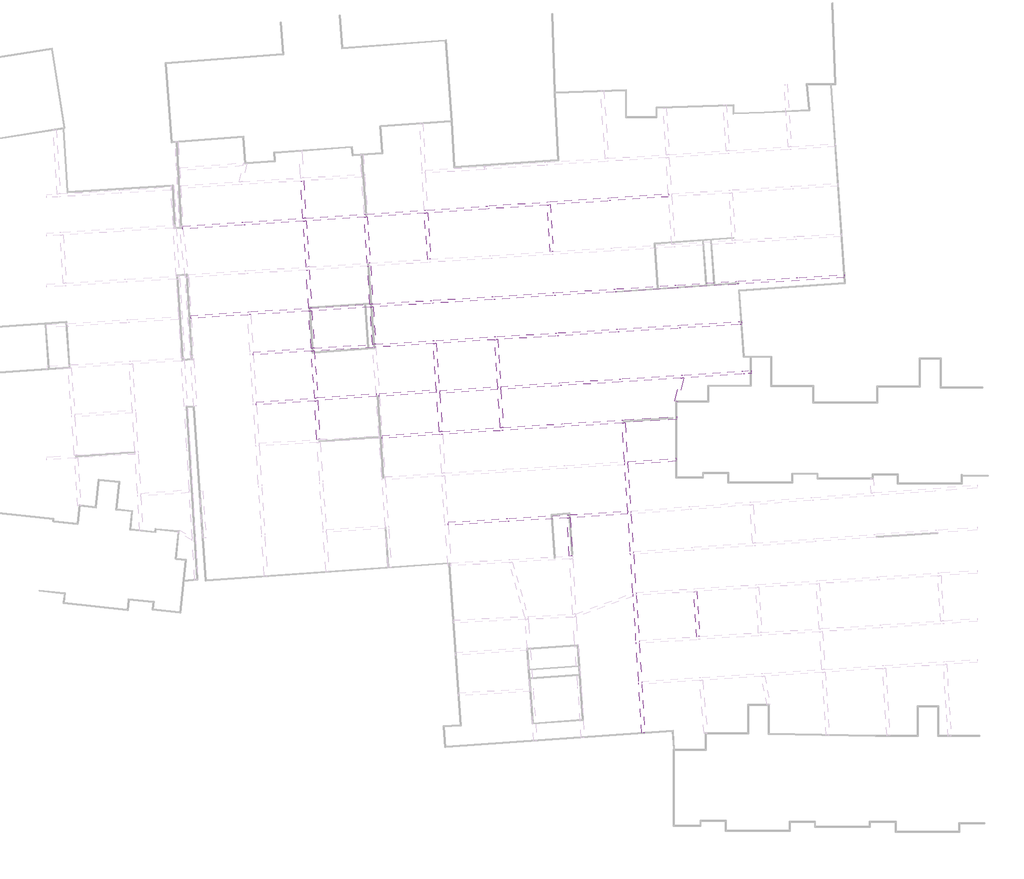
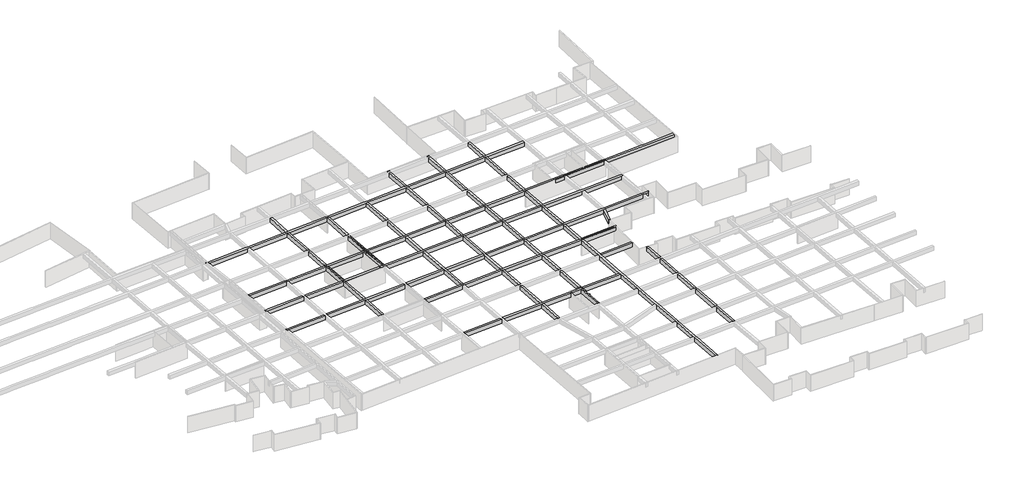
# One storey, part 13 of 14: 27 beams.
"""IFC4 building model written with IfcOpenShell, lengths in millimetres."""

from ifc_helpers import new_model, si_unit, frame, origin, place, context, project, spatial, polyline, outline, extrude, faceted_brep, element, save

model = new_model("IFC4")

# Units and contexts
model_context = context("Model", 3, world=origin())
ifc_project = project(units=[si_unit("LENGTHUNIT", "METRE", prefix="MILLI")], contexts=[model_context])

# Site, building, storey
site = spatial("IfcSite", under=ifc_project)
building = spatial("IfcBuilding", under=site)
storey = spatial("IfcBuildingStorey", under=building, Name="户型图", Elevation=0.0)

# Beams
placement = place(None, origin())
element("IfcBeam", 1, ObjectType="混凝土 - 矩形梁 : KL_beam", at=placement, inside=storey, context=model_context, shape_type="Brep", body=[
    faceted_brep([(-138257.4280169, -132256.5266916, 3300.0), (-138210.5692457, -132654.2910271, 3300.0), (-130469.1405666, -132138.3296148, 3300.0), (-130070.0241354, -132111.7287526, 3300.0), (-122474.0579494, -131605.462325, 3300.0), (-122074.9434283, -131578.8615901, 3300.0), (-114428.1793907, -131069.2095173, 3300.0), (-114029.0614384, -131042.6085537, 3300.0), (-106557.1829705, -130544.6124955, 3300.0), (-106158.0684495, -130518.0117606, 3300.0), (-98469.0899467, -130005.5461199, 3300.0), (-98069.9743702, -129978.9453146, 3300.0), (-90486.7784169, -129473.5300151, 3300.0), (-90087.6628405, -129446.9292099, 3300.0), (-82518.8955366, -128942.4755709, 3300.0), (-82119.7795402, -128915.8747377, 3300.0), (-74549.1899952, -128411.2996475, 3300.0), (-74577.0927331, -128012.2719042, 3300.0), (-82145.2950928, -128516.6878899, 3300.0), (-82544.4110892, -128543.2887232, 3300.0), (-90113.3457028, -129047.7535132, 3300.0), (-90512.4612793, -129074.3543185, 3300.0), (-98095.6572325, -129579.7696179, 3300.0), (-98494.772809, -129606.3704232, 3300.0), (-106181.8169664, -130118.707141, 3300.0), (-106580.971679, -130145.3105546, 3300.0), (-114054.8364044, -130643.4389957, 3300.0), (-114453.9509255, -130670.0397306, 3300.0), (-122098.6919453, -131179.5569705, 3300.0), (-122497.8466579, -131206.1603841, 3300.0), (-130095.3900507, -131712.5319316, 3300.0), (-130494.5064819, -131739.1327938, 3300.0), (-138244.7036771, -132255.6786223, 3300.0), (-138210.5692457, -132654.2910271, 2500.0), (-130469.1405666, -132138.3296148, 2500.0), (-130070.0241354, -132111.7287526, 2500.0), (-122474.0579494, -131605.462325, 2500.0), (-122074.9434283, -131578.8615901, 2500.0), (-114428.1793907, -131069.2095173, 2500.0), (-114029.0614384, -131042.6085537, 2500.0), (-106557.1829705, -130544.6124955, 2500.0), (-106158.0684495, -130518.0117606, 2500.0), (-98469.0899467, -130005.5461199, 2500.0), (-98069.9743702, -129978.9453146, 2500.0), (-90486.7784169, -129473.5300151, 2500.0), (-90087.6628405, -129446.9292099, 2500.0), (-82518.8955366, -128942.4755709, 2500.0), (-82119.7795402, -128915.8747377, 2500.0), (-74549.1899952, -128411.2996475, 2500.0), (-138257.4280169, -132256.5266916, 2500.0), (-138244.7036771, -132255.6786223, 2500.0), (-130494.5064819, -131739.1327938, 2500.0), (-130095.3900507, -131712.5319316, 2500.0), (-122497.8466579, -131206.1603841, 2500.0), (-122098.6919453, -131179.5569705, 2500.0), (-114453.9509255, -130670.0397306, 2500.0), (-114054.8364044, -130643.4389957, 2500.0), (-106580.971679, -130145.3105546, 2500.0), (-106181.8169664, -130118.707141, 2500.0), (-98494.772809, -129606.3704232, 2500.0), (-98095.6572325, -129579.7696179, 2500.0), (-90512.4612793, -129074.3543185, 2500.0), (-90113.3457028, -129047.7535132, 2500.0), (-82544.4110892, -128543.2887232, 2500.0), (-82145.2950928, -128516.6878899, 2500.0), (-74577.0927331, -128012.2719042, 2500.0), (-138657.0563303, -132283.1616705, 2500.0), (-138657.0563303, -132283.1616705, 3300.0), (-138643.8583896, -132282.2820359, 3300.0), (-138643.8583896, -132282.2820359, 2500.0), (-138654.6809564, -132303.3252176, 2500.0), (-138654.6809564, -132303.3252176, 3300.0)], [[[0, 1, 2, 3, 4, 5, 6, 7, 8, 9, 10, 11, 12, 13, 14, 15, 16, 17, 18, 19, 20, 21, 22, 23, 24, 25, 26, 27, 28, 29, 30, 31, 32]], [[1, 33, 34, 35, 36, 37, 38, 39, 40, 41, 42, 43, 44, 45, 46, 47, 48, 16, 15, 14, 13, 12, 11, 10, 9, 8, 7, 6, 5, 4, 3, 2]], [[33, 49, 50, 51, 52, 53, 54, 55, 56, 57, 58, 59, 60, 61, 62, 63, 64, 65, 48, 47, 46, 45, 44, 43, 42, 41, 40, 39, 38, 37, 36, 35, 34]], [[66, 67, 68, 0, 32, 31, 30, 29, 28, 27, 26, 25, 24, 23, 22, 21, 20, 19, 18, 17, 65, 64, 63, 62, 61, 60, 59, 58, 57, 56, 55, 54, 53, 52, 51, 50, 49, 69]], [[67, 66, 70, 71]], [[0, 49, 33, 1]], [[49, 0, 71, 70]], [[67, 71, 0, 68]], [[70, 66, 69, 49]], [[17, 16, 48, 65]]]),
])
element("IfcBeam", 2, ObjectType="混凝土 - 矩形梁 : KL_beam", at=placement, inside=storey, context=model_context, shape_type="Brep", body=[
    faceted_brep([(-51536.7180221, -138597.7306063, 3300.0), (-51511.7724706, -138996.9519979, 3300.0), (-51511.7724706, -138996.9519979, 2500.0), (-51536.7180221, -138597.7306063, 2500.0), (-57425.127004, -138965.6708341, 3300.0), (-57824.3483955, -138990.6163857, 3300.0), (-65411.3764652, -139464.6956904, 3300.0), (-65810.6088137, -139489.6419266, 3300.0), (-73340.6382748, -139960.1596443, 3300.0), (-73739.8706232, -139985.1058805, 3300.0), (-81381.7257688, -140462.611083, 3300.0), (-81780.9475672, -140487.5566599, 3300.0), (-89346.8943039, -140960.3186869, 3300.0), (-89746.1163762, -140985.2642809, 3300.0), (-97331.3357508, -141459.2305685, 3300.0), (-97730.5578232, -141484.1761625, 3300.0), (-105395.2598308, -141963.1089628, 3300.0), (-105794.4846545, -141988.0547288, 3300.0), (-113315.7632998, -142458.0256473, 3300.0), (-113714.9846914, -142482.9711989, 3300.0), (-121338.0144185, -142959.3000855, 3300.0), (-121737.2358101, -142984.245637, 3300.0), (-129348.9364688, -143459.8666211, 3300.0), (-129748.1580815, -143484.8121864, 3300.0), (-137166.9194829, -143948.3772629, 3300.0), (-137141.9739314, -144347.5986544, 3300.0), (-129722.7922736, -143884.007318, 3300.0), (-129323.5706608, -143859.0617527, 3300.0), (-121712.2902585, -143383.4670286, 3300.0), (-121313.068867, -143358.521477, 3300.0), (-113688.5657164, -142882.1005228, 3300.0), (-113289.333368, -142857.1542866, 3300.0), (-105767.8836909, -142387.1726811, 3300.0), (-105368.6588672, -142362.2269151, 3300.0), (-97704.874985, -141883.3514844, 3300.0), (-97305.6529126, -141858.4058903, 3300.0), (-89720.433538, -141384.4396028, 3300.0), (-89321.2114657, -141359.4940087, 3300.0), (-81755.4320829, -140886.7424389, 3300.0), (-81356.2102845, -140861.796862, 3300.0), (-73711.9672679, -140384.1424522, 3300.0), (-73312.7349195, -140359.196216, 3300.0), (-65782.7054584, -139888.6784983, 3300.0), (-65383.4731099, -139863.7322621, 3300.0), (-137141.9739314, -144347.5986544, 2500.0), (-129722.7922736, -143884.007318, 2500.0), (-129323.5706608, -143859.0617527, 2500.0), (-121712.2902585, -143383.4670286, 2500.0), (-121313.068867, -143358.521477, 2500.0), (-113688.5657164, -142882.1005228, 2500.0), (-113289.333368, -142857.1542866, 2500.0), (-105767.8836909, -142387.1726811, 2500.0), (-105368.6588672, -142362.2269151, 2500.0), (-97704.874985, -141883.3514844, 2500.0), (-97305.6529126, -141858.4058903, 2500.0), (-89720.433538, -141384.4396028, 2500.0), (-89321.2114657, -141359.4940087, 2500.0), (-81755.4320829, -140886.7424389, 2500.0), (-81356.2102845, -140861.796862, 2500.0), (-73711.9672679, -140384.1424522, 2500.0), (-73312.7349195, -140359.196216, 2500.0), (-65782.7054584, -139888.6784983, 2500.0), (-65383.4731099, -139863.7322621, 2500.0), (-137166.9194829, -143948.3772629, 2500.0), (-129748.1580815, -143484.8121864, 2500.0), (-129348.9364688, -143459.8666211, 2500.0), (-121737.2358101, -142984.245637, 2500.0), (-121338.0144185, -142959.3000855, 2500.0), (-113714.9846914, -142482.9711989, 2500.0), (-113315.7632998, -142458.0256473, 2500.0), (-105794.4846545, -141988.0547288, 2500.0), (-105395.2598308, -141963.1089628, 2500.0), (-97730.5578232, -141484.1761625, 2500.0), (-97331.3357508, -141459.2305685, 2500.0), (-89746.1163762, -140985.2642809, 2500.0), (-89346.8943039, -140960.3186869, 2500.0), (-81780.9475672, -140487.5566599, 2500.0), (-81381.7257688, -140462.611083, 2500.0), (-73739.8706232, -139985.1058805, 2500.0), (-73340.6382748, -139960.1596443, 2500.0), (-65810.6088137, -139489.6419266, 2500.0), (-65411.3764652, -139464.6956904, 2500.0), (-57824.3483955, -138990.6163857, 2500.0), (-57425.127004, -138965.6708341, 2500.0)], [[[0, 1, 2, 3]], [[1, 0, 4, 5, 6, 7, 8, 9, 10, 11, 12, 13, 14, 15, 16, 17, 18, 19, 20, 21, 22, 23, 24, 25, 26, 27, 28, 29, 30, 31, 32, 33, 34, 35, 36, 37, 38, 39, 40, 41, 42, 43]], [[2, 1, 43, 42, 41, 40, 39, 38, 37, 36, 35, 34, 33, 32, 31, 30, 29, 28, 27, 26, 25, 44, 45, 46, 47, 48, 49, 50, 51, 52, 53, 54, 55, 56, 57, 58, 59, 60, 61, 62]], [[3, 2, 62, 61, 60, 59, 58, 57, 56, 55, 54, 53, 52, 51, 50, 49, 48, 47, 46, 45, 44, 63, 64, 65, 66, 67, 68, 69, 70, 71, 72, 73, 74, 75, 76, 77, 78, 79, 80, 81, 82, 83]], [[0, 3, 83, 82, 81, 80, 79, 78, 77, 76, 75, 74, 73, 72, 71, 70, 69, 68, 67, 66, 65, 64, 63, 24, 23, 22, 21, 20, 19, 18, 17, 16, 15, 14, 13, 12, 11, 10, 9, 8, 7, 6, 5, 4]], [[25, 24, 63, 44]]]),
])
element("IfcBeam", 3, ObjectType="混凝土 - 矩形梁 : KL_beam", at=placement, inside=storey, context=model_context, shape_type="SweptSolid", body=[
    extrude(outline(polyline([(-120929.3613848, -155172.8834874), (-120530.2749819, -155144.9766476), (-120265.8728019, -160190.0707833), (-120665.0977944, -160215.3331772), (-120929.3613848, -155172.8834874)])), frame((0.0, 0.0, 2500.0), z_axis=(0.0, 0.0, 1.0), x_axis=(1.0, 0.0, 0.0)), (0.0, 0.0, 1.0), 800.0),
])
element("IfcBeam", 4, ObjectType="混凝土 - 矩形梁 : KL_beam", at=placement, inside=storey, context=model_context, shape_type="SweptSolid", body=[
    extrude(outline(polyline([(-121381.57776, -148656.6152208), (-120982.3454116, -148631.6689846), (-120554.8096294, -154745.715518), (-120953.8352495, -154773.6181075), (-121381.57776, -148656.6152208)])), frame((0.0, 0.0, 2500.0), z_axis=(0.0, 0.0, 1.0), x_axis=(1.0, 0.0, 0.0)), (0.0, 0.0, 1.0), 800.0),
])
element("IfcBeam", 5, ObjectType="混凝土 - 矩形梁 : KL_beam", at=placement, inside=storey, context=model_context, shape_type="SweptSolid", body=[
    extrude(outline(polyline([(-121712.2902585, -143383.4670286), (-121313.068867, -143358.521477), (-121008.5143401, -148232.5240364), (-121407.7357316, -148257.4695879), (-121712.2902585, -143383.4670286)])), frame((0.0, 0.0, 2500.0), z_axis=(0.0, 0.0, 1.0), x_axis=(1.0, 0.0, 0.0)), (0.0, 0.0, 1.0), 800.0),
])
element("IfcBeam", 6, ObjectType="混凝土 - 矩形梁 : KL_beam", at=placement, inside=storey, context=model_context, shape_type="SweptSolid", body=[
    extrude(outline(polyline([(-122048.4315655, -138003.9587776), (-121649.210174, -137979.0132261), (-121338.0144185, -142959.3000855), (-121737.2358101, -142984.245637), (-122048.4315655, -138003.9587776)])), frame((0.0, 0.0, 2500.0), z_axis=(0.0, 0.0, 1.0), x_axis=(1.0, 0.0, 0.0)), (0.0, 0.0, 1.0), 800.0),
])
element("IfcBeam", 7, ObjectType="混凝土 - 矩形梁 : KL_beam", at=placement, inside=storey, context=model_context, shape_type="SweptSolid", body=[
    extrude(outline(polyline([(-122474.0579494, -131605.462325), (-122074.9434283, -131578.8615901), (-121674.9817155, -137579.843447), (-122074.2065392, -137604.789213), (-122474.0579494, -131605.462325)])), frame((0.0, 0.0, 2500.0), z_axis=(0.0, 0.0, 1.0), x_axis=(1.0, 0.0, 0.0)), (0.0, 0.0, 1.0), 800.0),
])
element("IfcBeam", 8, ObjectType="混凝土 - 矩形梁 : KL_beam", at=placement, inside=storey, context=model_context, shape_type="SweptSolid", body=[
    extrude(outline(polyline([(-122098.6919453, -131179.5569705), (-122497.8466579, -131206.1603841), (-122753.4617992, -126328.7329342), (-122354.2077216, -126304.0255169), (-122098.6919453, -131179.5569705)])), frame((0.0, 0.0, 2500.0), z_axis=(0.0, 0.0, 1.0), x_axis=(1.0, 0.0, 0.0)), (0.0, 0.0, 1.0), 800.0),
])
element("IfcBeam", 9, ObjectType="混凝土 - 矩形梁 : KL_beam", at=placement, inside=storey, context=model_context, shape_type="SweptSolid", body=[
    extrude(outline(polyline([(-114428.1793907, -131069.2095173), (-114029.0614384, -131042.6085537), (-113651.9046068, -137078.5173964), (-114051.1259984, -137103.462948), (-114428.1793907, -131069.2095173)])), frame((0.0, 0.0, 2500.0), z_axis=(0.0, 0.0, 1.0), x_axis=(1.0, 0.0, 0.0)), (0.0, 0.0, 1.0), 800.0),
])
element("IfcBeam", 10, ObjectType="混凝土 - 矩形梁 : KL_beam", at=placement, inside=storey, context=model_context, shape_type="SweptSolid", body=[
    extrude(outline(polyline([(-114026.1804468, -137502.6843395), (-113626.9590553, -137477.738788), (-113315.7632998, -142458.0256473), (-113714.9846914, -142482.9711989), (-114026.1804468, -137502.6843395)])), frame((0.0, 0.0, 2500.0), z_axis=(0.0, 0.0, 1.0), x_axis=(1.0, 0.0, 0.0)), (0.0, 0.0, 1.0), 800.0),
])
element("IfcBeam", 11, ObjectType="混凝土 - 矩形梁 : KL_beam", at=placement, inside=storey, context=model_context, shape_type="SweptSolid", body=[
    extrude(outline(polyline([(-113688.5657164, -142882.1005228), (-113289.333368, -142857.1542866), (-112948.6676921, -147728.9004225), (-113347.9000405, -147753.8466587), (-113688.5657164, -142882.1005228)])), frame((0.0, 0.0, 2500.0), z_axis=(0.0, 0.0, 1.0), x_axis=(1.0, 0.0, 0.0)), (0.0, 0.0, 1.0), 800.0),
])
element("IfcBeam", 12, ObjectType="混凝土 - 矩形梁 : KL_beam", at=placement, inside=storey, context=model_context, shape_type="Brep", body=[
    faceted_brep([(-105016.5352555, -147634.037223, 3300.0), (-105415.767604, -147658.9834592, 3300.0), (-104996.292424, -153657.7580113, 3300.0), (-104968.3898345, -154056.7836314, 3300.0), (-104609.2265906, -159193.0573148, 3300.0), (-104210.0389543, -159167.4716642, 3300.0), (-104555.4129197, -154228.3938519, 3300.0), (-104583.3155091, -153829.3682318, 3300.0), (-105016.5352555, -147634.037223, 2500.0), (-104210.0389543, -159167.4716642, 2500.0), (-104555.4129197, -154228.3938519, 2500.0), (-104583.3155091, -153829.3682318, 2500.0), (-105415.767604, -147658.9834592, 2500.0), (-104609.2265906, -159193.0573148, 2500.0), (-104968.3898345, -154056.7836314, 2500.0), (-104996.292424, -153657.7580113, 2500.0)], [[[0, 1, 2, 3, 4, 5, 6, 7]], [[8, 0, 7, 6, 5, 9, 10, 11]], [[12, 8, 11, 10, 9, 13, 14, 15]], [[1, 12, 15, 14, 13, 4, 3, 2]], [[1, 0, 8, 12]], [[4, 13, 9, 5]]]),
])
element("IfcBeam", 13, ObjectType="混凝土 - 矩形梁 : KL_beam", at=placement, inside=storey, context=model_context, shape_type="SweptSolid", body=[
    extrude(outline(polyline([(-105043.8937937, -147234.9666081), (-105443.1186174, -147259.9123741), (-105767.8836909, -142387.1726811), (-105368.6588672, -142362.2269151), (-105043.8937937, -147234.9666081)])), frame((0.0, 0.0, 2500.0), z_axis=(0.0, 0.0, 1.0), x_axis=(1.0, 0.0, 0.0)), (0.0, 0.0, 1.0), 800.0),
    extrude(outline(polyline([(-106557.1829705, -130544.6124955), (-106158.0684495, -130518.0117606), (-105753.707815, -136584.9945559), (-106152.9326387, -136609.9403219), (-106557.1829705, -130544.6124955)])), frame((0.0, 0.0, 2500.0), z_axis=(0.0, 0.0, 1.0), x_axis=(1.0, 0.0, 0.0)), (0.0, 0.0, 1.0), 800.0),
    extrude(outline(polyline([(-106126.3316752, -137009.0582742), (-105727.1068515, -136984.1125082), (-105395.2598308, -141963.1089628), (-105794.4846545, -141988.0547288), (-106126.3316752, -137009.0582742)])), frame((0.0, 0.0, 2500.0), z_axis=(0.0, 0.0, 1.0), x_axis=(1.0, 0.0, 0.0)), (0.0, 0.0, 1.0), 800.0),
])
element("IfcBeam", 14, ObjectType="混凝土 - 矩形梁 : KL_beam", at=placement, inside=storey, context=model_context, shape_type="Brep", body=[
    faceted_brep([(-65016.908121, -144733.8600662, 3300.0), (-64991.9625695, -145133.0814577, 3300.0), (-64991.9625695, -145133.0814577, 2500.0), (-65016.908121, -144733.8600662, 2500.0), (-65042.807434, -144735.4783979, 3300.0), (-65442.0397825, -144760.4246341, 3300.0), (-72972.0692436, -145230.9423519, 3300.0), (-73371.301592, -145255.888588, 3300.0), (-81044.6975793, -145735.364636, 3300.0), (-81443.9193776, -145760.310213, 3300.0), (-89007.6555748, -146232.9341132, 3300.0), (-89406.8776471, -146257.8797073, 3300.0), (-96992.0970218, -146731.8459948, 3300.0), (-97391.3190941, -146756.7915889, 3300.0), (-105043.8937937, -147234.9666081, 3300.0), (-105443.1186174, -147259.9123741, 3300.0), (-112948.6676921, -147728.9004225, 3300.0), (-113347.9000405, -147753.8466587, 3300.0), (-121008.5143401, -148232.5240364, 3300.0), (-121407.7357316, -148257.4695879, 3300.0), (-129013.8853194, -148732.7437105, 3300.0), (-128988.5195114, -149131.9388421, 3300.0), (-121381.57776, -148656.6152208, 3300.0), (-120982.3454116, -148631.6689846, 3300.0), (-113319.9966852, -148152.8832303, 3300.0), (-112920.7643368, -148127.9369941, 3300.0), (-105415.767604, -147658.9834592, 3300.0), (-105016.5352555, -147634.037223, 3300.0), (-97365.6362559, -147155.9669107, 3300.0), (-96966.4141836, -147131.0213166, 3300.0), (-89381.1948089, -146657.0550291, 3300.0), (-88981.9727366, -146632.109435, 3300.0), (-81418.4038933, -146159.495992, 3300.0), (-81019.182095, -146134.550415, 3300.0), (-73343.3982367, -145654.9251597, 3300.0), (-72944.1658883, -145629.9789235, 3300.0), (-65414.1364272, -145159.4612058, 3300.0), (-65014.9040787, -145134.5149696, 3300.0), (-128988.5195114, -149131.9388421, 2500.0), (-121381.57776, -148656.6152208, 2500.0), (-120982.3454116, -148631.6689846, 2500.0), (-113319.9966852, -148152.8832303, 2500.0), (-112920.7643368, -148127.9369941, 2500.0), (-105415.767604, -147658.9834592, 2500.0), (-105016.5352555, -147634.037223, 2500.0), (-97365.6362559, -147155.9669107, 2500.0), (-96966.4141836, -147131.0213166, 2500.0), (-89381.1948089, -146657.0550291, 2500.0), (-88981.9727366, -146632.109435, 2500.0), (-81418.4038933, -146159.495992, 2500.0), (-81019.182095, -146134.550415, 2500.0), (-73343.3982367, -145654.9251597, 2500.0), (-72944.1658883, -145629.9789235, 2500.0), (-65414.1364272, -145159.4612058, 2500.0), (-65014.9040787, -145134.5149696, 2500.0), (-129013.8853194, -148732.7437105, 2500.0), (-121407.7357316, -148257.4695879, 2500.0), (-121008.5143401, -148232.5240364, 2500.0), (-113347.9000405, -147753.8466587, 2500.0), (-112948.6676921, -147728.9004225, 2500.0), (-105443.1186174, -147259.9123741, 2500.0), (-105043.8937937, -147234.9666081, 2500.0), (-97391.3190941, -146756.7915889, 2500.0), (-96992.0970218, -146731.8459948, 2500.0), (-89406.8776471, -146257.8797073, 2500.0), (-89007.6555748, -146232.9341132, 2500.0), (-81443.9193776, -145760.310213, 2500.0), (-81044.6975793, -145735.364636, 2500.0), (-73371.301592, -145255.888588, 2500.0), (-72972.0692436, -145230.9423519, 2500.0), (-65442.0397825, -144760.4246341, 2500.0), (-65042.807434, -144735.4783979, 2500.0)], [[[0, 1, 2, 3]], [[1, 0, 4, 5, 6, 7, 8, 9, 10, 11, 12, 13, 14, 15, 16, 17, 18, 19, 20, 21, 22, 23, 24, 25, 26, 27, 28, 29, 30, 31, 32, 33, 34, 35, 36, 37]], [[2, 1, 37, 36, 35, 34, 33, 32, 31, 30, 29, 28, 27, 26, 25, 24, 23, 22, 21, 38, 39, 40, 41, 42, 43, 44, 45, 46, 47, 48, 49, 50, 51, 52, 53, 54]], [[3, 2, 54, 53, 52, 51, 50, 49, 48, 47, 46, 45, 44, 43, 42, 41, 40, 39, 38, 55, 56, 57, 58, 59, 60, 61, 62, 63, 64, 65, 66, 67, 68, 69, 70, 71]], [[0, 3, 71, 70, 69, 68, 67, 66, 65, 64, 63, 62, 61, 60, 59, 58, 57, 56, 55, 20, 19, 18, 17, 16, 15, 14, 13, 12, 11, 10, 9, 8, 7, 6, 5, 4]], [[21, 20, 55, 38]]]),
    faceted_brep([(-137045.4296351, -149234.5988387, 3300.0), (-137045.4296351, -149234.5988387, 2500.0), (-137020.4840836, -149633.8202303, 2500.0), (-137020.4840836, -149633.8202303, 3300.0), (-129413.1069321, -148757.6892758, 3300.0), (-129387.7411242, -149156.8844074, 3300.0), (-129387.7411242, -149156.8844074, 2500.0), (-129413.1069321, -148757.6892758, 2500.0), (-136812.4738529, -149620.8226053, 3300.0), (-136837.4194044, -149221.6012138, 3300.0), (-136812.4738529, -149620.8226053, 2500.0), (-136837.4194044, -149221.6012138, 2500.0)], [[[0, 1, 2, 3]], [[4, 5, 6, 7]], [[0, 3, 8, 5, 4, 9]], [[3, 2, 10, 6, 5, 8]], [[2, 1, 11, 7, 6, 10]], [[1, 0, 9, 4, 7, 11]]]),
])
element("IfcBeam", 15, ObjectType="混凝土 - 矩形梁 : KL_beam", at=placement, inside=storey, context=model_context, shape_type="Brep", body=[
    faceted_brep([(-136811.0666065, -155882.4637426, 3300.0), (-136811.0666065, -155882.4637426, 2500.0), (-136783.164017, -156281.4893627, 2500.0), (-136783.164017, -156281.4893627, 3300.0), (-128995.1105813, -155335.9188554, 3300.0), (-128969.744275, -155735.1218297, 3300.0), (-128969.744275, -155735.1218297, 2500.0), (-128995.1105813, -155335.9188554, 2500.0), (-136757.1148251, -156279.6678257, 3300.0), (-136358.089205, -156251.7652362, 3300.0), (-136385.9917945, -155852.7396161, 3300.0), (-136785.0174146, -155880.6422056, 3300.0), (-136757.1148251, -156279.6678257, 2500.0), (-136358.089205, -156251.7652362, 2500.0), (-136785.0174146, -155880.6422056, 2500.0), (-136385.9917945, -155852.7396161, 2500.0)], [[[0, 1, 2, 3]], [[4, 5, 6, 7]], [[0, 3, 8, 9, 5, 4, 10, 11]], [[3, 2, 12, 13, 6, 5, 9, 8]], [[2, 1, 14, 15, 7, 6, 13, 12]], [[1, 0, 11, 10, 4, 7, 15, 14]]]),
    faceted_brep([(-112868.5259901, -154609.2149667, 3300.0), (-112896.4285796, -154210.1893466, 3300.0), (-120554.8096294, -154745.715518, 3300.0), (-120953.8352495, -154773.6181075, 3300.0), (-128596.0769007, -155308.0157023, 3300.0), (-128570.7105944, -155707.2186766, 3300.0), (-120929.3613848, -155172.8834874, 3300.0), (-120530.2749819, -155144.9766476, 3300.0), (-112868.5259901, -154609.2149667, 2500.0), (-128570.7105944, -155707.2186766, 2500.0), (-120929.3613848, -155172.8834874, 2500.0), (-120530.2749819, -155144.9766476, 2500.0), (-112896.4285796, -154210.1893466, 2500.0), (-128596.0769007, -155308.0157023, 2500.0), (-120953.8352495, -154773.6181075, 2500.0), (-120554.8096294, -154745.715518, 2500.0)], [[[0, 1, 2, 3, 4, 5, 6, 7]], [[8, 0, 7, 6, 5, 9, 10, 11]], [[12, 8, 11, 10, 9, 13, 14, 15]], [[1, 12, 15, 14, 13, 4, 3, 2]], [[1, 0, 8, 12]], [[5, 4, 13, 9]]]),
])
element("IfcBeam", 16, ObjectType="混凝土 - 矩形梁 : KL_beam", at=placement, inside=storey, context=model_context, shape_type="SweptSolid", body=[
    extrude(outline(polyline([(-112469.50037, -154581.3123772), (-112497.4029595, -154182.2867571), (-104996.292424, -153657.7580113), (-104968.3898345, -154056.7836314), (-112469.50037, -154581.3123772)])), frame((0.0, 0.0, 2500.0), z_axis=(0.0, 0.0, 1.0), x_axis=(1.0, 0.0, 0.0)), (0.0, 0.0, 1.0), 800.0),
])
element("IfcBeam", 17, ObjectType="混凝土 - 矩形梁 : KL_beam", at=placement, inside=storey, context=model_context, shape_type="SweptSolid", body=[
    extrude(outline(polyline([(-104555.4129197, -154228.3938519), (-104583.3155091, -153829.3682318), (-96970.5218364, -153297.0298403), (-96944.8386448, -153696.2106558), (-104555.4129197, -154228.3938519)])), frame((0.0, 0.0, 2500.0), z_axis=(0.0, 0.0, 1.0), x_axis=(1.0, 0.0, 0.0)), (0.0, 0.0, 1.0), 800.0),
])
element("IfcBeam", 18, ObjectType="混凝土 - 矩形梁 : KL_beam", at=placement, inside=storey, context=model_context, shape_type="Brep", body=[
    faceted_brep([(-63719.3871794, -151179.7439422, 3300.0), (-63693.9811028, -151578.9362909, 3300.0), (-63693.9811028, -151578.9362909, 2500.0), (-63719.3871794, -151179.7439422, 2500.0), (-64588.3134192, -151235.04562, 3300.0), (-64987.5135777, -151260.4521937, 3300.0), (-72516.9358957, -151739.652462, 3300.0), (-72916.1360542, -151765.0590358, 3300.0), (-80627.9148756, -152255.865146, 3300.0), (-81027.1072393, -152281.2712237, 3300.0), (-88587.5484712, -152762.4456504, 3300.0), (-88986.7409158, -152787.8517331, 3300.0), (-96571.3973636, -153270.5673057, 3300.0), (-96545.7145631, -153669.7420426, 3300.0), (-88961.0581152, -153187.0264701, 3300.0), (-88561.8656706, -153161.6203873, 3300.0), (-81001.59178, -152680.4566109, 3300.0), (-80602.3994163, -152655.0505332, 3300.0), (-72967.8617536, -152169.1603358, 3300.0), (-72546.5668223, -152142.3475691, 3300.0), (-64959.6104423, -151659.4856204, 3300.0), (-64560.4102838, -151634.0790467, 3300.0), (-96545.7145631, -153669.7420426, 2500.0), (-88961.0581152, -153187.0264701, 2500.0), (-88561.8656706, -153161.6203873, 2500.0), (-81001.59178, -152680.4566109, 2500.0), (-80602.3994163, -152655.0505332, 2500.0), (-72967.8617536, -152169.1603358, 2500.0), (-72546.5668223, -152142.3475691, 2500.0), (-64959.6104423, -151659.4856204, 2500.0), (-64560.4102838, -151634.0790467, 2500.0), (-96571.3973636, -153270.5673057, 2500.0), (-88986.7409158, -152787.8517331, 2500.0), (-88587.5484712, -152762.4456504, 2500.0), (-81027.1072393, -152281.2712237, 2500.0), (-80627.9148756, -152255.865146, 2500.0), (-72916.1360542, -151765.0590358, 2500.0), (-72516.9358957, -151739.652462, 2500.0), (-64987.5135777, -151260.4521937, 2500.0), (-64588.3134192, -151235.04562, 2500.0)], [[[0, 1, 2, 3]], [[1, 0, 4, 5, 6, 7, 8, 9, 10, 11, 12, 13, 14, 15, 16, 17, 18, 19, 20, 21]], [[2, 1, 21, 20, 19, 18, 17, 16, 15, 14, 13, 22, 23, 24, 25, 26, 27, 28, 29, 30]], [[3, 2, 30, 29, 28, 27, 26, 25, 24, 23, 22, 31, 32, 33, 34, 35, 36, 37, 38, 39]], [[0, 3, 39, 38, 37, 36, 35, 34, 33, 32, 31, 12, 11, 10, 9, 8, 7, 6, 5, 4]], [[12, 31, 22, 13]]]),
])
element("IfcBeam", 19, ObjectType="混凝土 - 矩形梁 : KL_beam", at=placement, inside=storey, context=model_context, shape_type="Brep", body=[
    faceted_brep([(-73511.9550668, -157199.8995786, 3300.0), (-73486.3698475, -157599.0804856, 3300.0), (-73486.3698475, -157599.0804856, 2500.0), (-73511.9550668, -157199.8995786, 2500.0), (-80284.1534665, -157633.9588697, 3300.0), (-80683.3343797, -157659.5440894, 3300.0), (-88241.3027785, -158143.9667556, 3300.0), (-88640.4836975, -158169.5519758, 3300.0), (-96224.921158, -158655.6711579, 3300.0), (-96624.102077, -158681.256378, 3300.0), (-104210.0389543, -159167.4716642, 3300.0), (-104609.2265906, -159193.0573148, 3300.0), (-112113.3827977, -159674.0309265, 3300.0), (-112085.4797378, -160073.0632732, 3300.0), (-104584.7031482, -159592.3062757, 3300.0), (-104185.4951653, -159566.719321, 3300.0), (-96598.4192818, -159080.431031, 3300.0), (-96199.2383628, -159054.8458109, 3300.0), (-88614.8009023, -158568.7266287, 3300.0), (-88215.6199834, -158543.1414086, 3300.0), (-80657.818921, -158058.7294677, 3300.0), (-80258.6380079, -158033.144248, 3300.0), (-112085.4797378, -160073.0632732, 2500.0), (-104584.7031482, -159592.3062757, 2500.0), (-104185.4951653, -159566.719321, 2500.0), (-96598.4192818, -159080.431031, 2500.0), (-96199.2383628, -159054.8458109, 2500.0), (-88614.8009023, -158568.7266287, 2500.0), (-88215.6199834, -158543.1414086, 2500.0), (-80657.818921, -158058.7294677, 2500.0), (-80258.6380079, -158033.144248, 2500.0), (-112113.3827977, -159674.0309265, 2500.0), (-104609.2265906, -159193.0573148, 2500.0), (-104210.0389543, -159167.4716642, 2500.0), (-96624.102077, -158681.256378, 2500.0), (-96224.921158, -158655.6711579, 2500.0), (-88640.4836975, -158169.5519758, 2500.0), (-88241.3027785, -158143.9667556, 2500.0), (-80683.3343797, -157659.5440894, 2500.0), (-80284.1534665, -157633.9588697, 2500.0)], [[[0, 1, 2, 3]], [[1, 0, 4, 5, 6, 7, 8, 9, 10, 11, 12, 13, 14, 15, 16, 17, 18, 19, 20, 21]], [[2, 1, 21, 20, 19, 18, 17, 16, 15, 14, 13, 22, 23, 24, 25, 26, 27, 28, 29, 30]], [[3, 2, 30, 29, 28, 27, 26, 25, 24, 23, 22, 31, 32, 33, 34, 35, 36, 37, 38, 39]], [[0, 3, 39, 38, 37, 36, 35, 34, 33, 32, 31, 12, 11, 10, 9, 8, 7, 6, 5, 4]], [[13, 12, 31, 22]]]),
])
element("IfcBeam", 20, ObjectType="混凝土 - 矩形梁 : KL_beam", at=placement, inside=storey, context=model_context, shape_type="SweptSolid", body=[
    extrude(outline(polyline([(-73597.9130009, -162674.974788), (-73570.0104114, -163074.0004082), (-79908.1034361, -163517.2030472), (-79933.6193508, -163118.0105345), (-73597.9130009, -162674.974788)])), frame((0.0, 0.0, 2500.0), z_axis=(0.0, 0.0, 1.0), x_axis=(1.0, 0.0, 0.0)), (0.0, 0.0, 1.0), 800.0),
])
element("IfcBeam", 21, ObjectType="混凝土 - 矩形梁 : KL_beam", at=placement, inside=storey, context=model_context, shape_type="Brep", body=[
    faceted_brep([(-103471.1509319, -171060.0722772, 3300.0), (-103443.2472635, -171459.1133269, 3300.0), (-95831.8970272, -170994.0974778, 3300.0), (-95432.6393797, -170969.7048105, 3300.0), (-87848.0262284, -170506.3224651, 3300.0), (-87448.7686337, -170481.9298011, 3300.0), (-79893.2478488, -170020.3248553, 3300.0), (-79918.763408, -169621.137904, 3300.0), (-87473.1693579, -170082.6747388, 3300.0), (-87872.4270054, -170107.0674061, 3300.0), (-95458.3223083, -170570.5280846, 3300.0), (-95857.5799558, -170594.9207519, 3300.0), (-103443.2472635, -171459.1133269, 2500.0), (-95831.8970272, -170994.0974778, 2500.0), (-95432.6393797, -170969.7048105, 2500.0), (-87848.0262284, -170506.3224651, 2500.0), (-87448.7686337, -170481.9298011, 2500.0), (-79893.2478488, -170020.3248553, 2500.0), (-103471.1509319, -171060.0722772, 2500.0), (-95857.5799558, -170594.9207519, 2500.0), (-95458.3223083, -170570.5280846, 2500.0), (-87872.4270054, -170107.0674061, 2500.0), (-87473.1693579, -170082.6747388, 2500.0), (-79918.763408, -169621.137904, 2500.0)], [[[0, 1, 2, 3, 4, 5, 6, 7, 8, 9, 10, 11]], [[1, 12, 13, 14, 15, 16, 17, 6, 5, 4, 3, 2]], [[12, 18, 19, 20, 21, 22, 23, 17, 16, 15, 14, 13]], [[18, 0, 11, 10, 9, 8, 7, 23, 22, 21, 20, 19]], [[1, 0, 18, 12]], [[7, 6, 17, 23]]]),
    faceted_brep([(-111255.912427, -171936.4285221, 3300.0), (-111283.8160955, -171537.3874725, 3300.0), (-111283.8160955, -171537.3874725, 2500.0), (-111255.912427, -171936.4285221, 2500.0), (-103870.4219326, -171084.4657603, 3300.0), (-103842.5182642, -171483.50681, 3300.0), (-103842.5182642, -171483.50681, 2500.0), (-103870.4219326, -171084.4657603, 2500.0)], [[[0, 1, 2, 3]], [[4, 5, 6, 7]], [[1, 0, 5, 4]], [[0, 3, 6, 5]], [[3, 2, 7, 6]], [[2, 1, 4, 7]]]),
])
element("IfcBeam", 22, ObjectType="混凝土 - 矩形梁 : KL_beam", at=placement, inside=storey, context=model_context, shape_type="SweptSolid", body=[
    extrude(outline(polyline([(-73390.2802922, -155291.129106), (-73776.6506227, -155187.601488), (-72967.8617536, -152169.1603358), (-72546.5668223, -152142.3475691), (-73390.2802922, -155291.129106)])), frame((0.0, 0.0, 2500.0), z_axis=(0.0, 0.0, 1.0), x_axis=(1.0, 0.0, 0.0)), (0.0, 0.0, 1.0), 800.0),
])
element("IfcBeam", 23, ObjectType="混凝土 - 矩形梁 : KL_beam", at=placement, inside=storey, context=model_context, shape_type="Brep", body=[
    faceted_brep([(-77660.3791239, -198682.49996, 3300.0), (-78059.5644962, -198708.0154183, 3300.0), (-78059.5644962, -198708.0154183, 2500.0), (-77660.3791239, -198682.49996, 2500.0), (-78066.8659891, -192323.0762413, 3300.0), (-78092.3814613, -191923.8906508, 3300.0), (-78408.7670142, -186974.087934, 3300.0), (-78434.2824865, -186574.9023435, 3300.0), (-78810.9634026, -180681.7880572, 3300.0), (-78836.4788748, -180282.6024667, 3300.0), (-79154.5618568, -175306.243736, 3300.0), (-79180.0779467, -174907.0484814, 3300.0), (-79494.0977596, -169994.2573993, 3300.0), (-79519.6147606, -169595.0478922, 3300.0), (-79908.1034361, -163517.2030472, 3300.0), (-79933.6193508, -163118.0105345, 3300.0), (-80258.6380079, -158033.144248, 3300.0), (-80657.818921, -158058.7294677, 3300.0), (-80332.7790985, -163143.9268851, 3300.0), (-80307.2636103, -163543.1127259, 3300.0), (-79918.763408, -169621.137904, 3300.0), (-79893.2478488, -170020.3248553, 3300.0), (-79579.0837782, -174935.3728265, 3300.0), (-79553.5676883, -175334.5680811, 3300.0), (-79232.4471215, -180358.4493525, 3300.0), (-79205.8573257, -180774.4425673, 3300.0), (-78833.4545077, -186600.626675, 3300.0), (-78807.9390495, -186999.8120473, 3300.0), (-78491.5534826, -191949.6149824, 3300.0), (-78466.0380243, -192348.8003546, 3300.0), (-80657.818921, -158058.7294677, 2500.0), (-80332.7790985, -163143.9268851, 2500.0), (-80307.2636103, -163543.1127259, 2500.0), (-79918.763408, -169621.137904, 2500.0), (-79893.2478488, -170020.3248553, 2500.0), (-79579.0837782, -174935.3728265, 2500.0), (-79553.5676883, -175334.5680811, 2500.0), (-79232.4471215, -180358.4493525, 2500.0), (-79205.8573257, -180774.4425673, 2500.0), (-78833.4545077, -186600.626675, 2500.0), (-78807.9390495, -186999.8120473, 2500.0), (-78491.5534826, -191949.6149824, 2500.0), (-78466.0380243, -192348.8003546, 2500.0), (-80258.6380079, -158033.144248, 2500.0), (-79933.6193508, -163118.0105345, 2500.0), (-79908.1034361, -163517.2030472, 2500.0), (-79519.6147606, -169595.0478922, 2500.0), (-79494.0977596, -169994.2573993, 2500.0), (-79180.0779467, -174907.0484814, 2500.0), (-79154.5618568, -175306.243736, 2500.0), (-78836.4788748, -180282.6024667, 2500.0), (-78810.9634026, -180681.7880572, 2500.0), (-78434.2824865, -186574.9023435, 2500.0), (-78408.7670142, -186974.087934, 2500.0), (-78092.3814613, -191923.8906508, 2500.0), (-78066.8659891, -192323.0762413, 2500.0)], [[[0, 1, 2, 3]], [[1, 0, 4, 5, 6, 7, 8, 9, 10, 11, 12, 13, 14, 15, 16, 17, 18, 19, 20, 21, 22, 23, 24, 25, 26, 27, 28, 29]], [[2, 1, 29, 28, 27, 26, 25, 24, 23, 22, 21, 20, 19, 18, 17, 30, 31, 32, 33, 34, 35, 36, 37, 38, 39, 40, 41, 42]], [[3, 2, 42, 41, 40, 39, 38, 37, 36, 35, 34, 33, 32, 31, 30, 43, 44, 45, 46, 47, 48, 49, 50, 51, 52, 53, 54, 55]], [[0, 3, 55, 54, 53, 52, 51, 50, 49, 48, 47, 46, 45, 44, 43, 16, 15, 14, 13, 12, 11, 10, 9, 8, 7, 6, 5, 4]], [[17, 16, 43, 30]]]),
    faceted_brep([(-82849.1027592, -123776.4349832, 3300.0), (-82449.9129148, -123750.9894916, 3300.0), (-82449.9129148, -123750.9894916, 2500.0), (-82849.1027592, -123776.4349832, 2500.0), (-82145.2950928, -128516.6878899, 3300.0), (-82544.4110892, -128543.2887232, 3300.0), (-82544.4110892, -128543.2887232, 2500.0), (-82145.2950928, -128516.6878899, 2500.0)], [[[0, 1, 2, 3]], [[4, 5, 6, 7]], [[1, 0, 5, 4]], [[0, 3, 6, 5]], [[3, 2, 7, 6]], [[2, 1, 4, 7]]]),
    faceted_brep([(-82518.8955366, -128942.4755709, 3300.0), (-82119.7795402, -128915.8747377, 3300.0), (-82119.7795402, -128915.8747377, 2500.0), (-82518.8955366, -128942.4755709, 2500.0), (-81725.5469195, -135083.582711, 3300.0), (-82124.7687178, -135108.5282879, 3300.0), (-82124.7687178, -135108.5282879, 2500.0), (-81725.5469195, -135083.582711, 2500.0)], [[[0, 1, 2, 3]], [[4, 5, 6, 7]], [[1, 0, 5, 4]], [[0, 3, 6, 5]], [[3, 2, 7, 6]], [[2, 1, 4, 7]]]),
    faceted_brep([(-82099.2532336, -135507.7140669, 3300.0), (-81700.0314352, -135482.76849, 3300.0), (-81700.0314352, -135482.76849, 2500.0), (-82099.2532336, -135507.7140669, 2500.0), (-81381.7257688, -140462.611083, 3300.0), (-81780.9475672, -140487.5566599, 3300.0), (-81780.9475672, -140487.5566599, 2500.0), (-81381.7257688, -140462.611083, 2500.0)], [[[0, 1, 2, 3]], [[4, 5, 6, 7]], [[1, 0, 5, 4]], [[0, 3, 6, 5]], [[3, 2, 7, 6]], [[2, 1, 4, 7]]]),
    faceted_brep([(-81755.4320829, -140886.7424389, 3300.0), (-81356.2102845, -140861.796862, 3300.0), (-81356.2102845, -140861.796862, 2500.0), (-81755.4320829, -140886.7424389, 2500.0), (-81044.6975793, -145735.364636, 3300.0), (-81443.9193776, -145760.310213, 3300.0), (-81443.9193776, -145760.310213, 2500.0), (-81044.6975793, -145735.364636, 2500.0)], [[[0, 1, 2, 3]], [[4, 5, 6, 7]], [[1, 0, 5, 4]], [[0, 3, 6, 5]], [[3, 2, 7, 6]], [[2, 1, 4, 7]]]),
    faceted_brep([(-81418.4038933, -146159.495992, 3300.0), (-81019.182095, -146134.550415, 3300.0), (-81019.182095, -146134.550415, 2500.0), (-81418.4038933, -146159.495992, 2500.0), (-80627.9148756, -152255.865146, 3300.0), (-81027.1072393, -152281.2712237, 3300.0), (-81027.1072393, -152281.2712237, 2500.0), (-80627.9148756, -152255.865146, 2500.0)], [[[0, 1, 2, 3]], [[4, 5, 6, 7]], [[1, 0, 5, 4]], [[0, 3, 6, 5]], [[3, 2, 7, 6]], [[2, 1, 4, 7]]]),
    faceted_brep([(-81001.59178, -152680.4566109, 3300.0), (-80602.3994163, -152655.0505332, 3300.0), (-80602.3994163, -152655.0505332, 2500.0), (-81001.59178, -152680.4566109, 2500.0), (-80284.1534665, -157633.9588697, 3300.0), (-80683.3343797, -157659.5440894, 3300.0), (-80683.3343797, -157659.5440894, 2500.0), (-80284.1534665, -157633.9588697, 2500.0)], [[[0, 1, 2, 3]], [[4, 5, 6, 7]], [[1, 0, 5, 4]], [[0, 3, 6, 5]], [[3, 2, 7, 6]], [[2, 1, 4, 7]]]),
])
element("IfcBeam", 24, ObjectType="混凝土 - 矩形梁 : KL_beam", at=placement, inside=storey, context=model_context, shape_type="SweptSolid", body=[
    extrude(outline(polyline([(-90856.9252889, -123720.5250084), (-90457.7506478, -123694.842214), (-90447.1281157, -123859.9428397), (-90846.3180245, -123885.3883354), (-90856.9252889, -123720.5250084)])), frame((0.0, 0.0, 2500.0), z_axis=(0.0, 0.0, 1.0), x_axis=(1.0, 0.0, 0.0)), (0.0, 0.0, 1.0), 800.0),
    extrude(outline(polyline([(-87473.1693579, -170082.6747388), (-87872.4270054, -170107.0674061), (-88262.8201611, -164039.3846846), (-87863.5954035, -164014.4808264), (-87473.1693579, -170082.6747388)])), frame((0.0, 0.0, 2500.0), z_axis=(0.0, 0.0, 1.0), x_axis=(1.0, 0.0, 0.0)), (0.0, 0.0, 1.0), 800.0),
    extrude(outline(polyline([(-90486.7784169, -129473.5300151), (-90087.6628405, -129446.9292099), (-89692.9705485, -135581.4312256), (-90092.1926208, -135606.3768197), (-90486.7784169, -129473.5300151)])), frame((0.0, 0.0, 2500.0), z_axis=(0.0, 0.0, 1.0), x_axis=(1.0, 0.0, 0.0)), (0.0, 0.0, 1.0), 800.0),
    extrude(outline(polyline([(-90113.3457028, -129047.7535132), (-90512.4612793, -129074.3543185), (-90820.6352256, -124284.563047), (-90421.4453168, -124259.1175513), (-90113.3457028, -129047.7535132)])), frame((0.0, 0.0, 2500.0), z_axis=(0.0, 0.0, 1.0), x_axis=(1.0, 0.0, 0.0)), (0.0, 0.0, 1.0), 800.0),
    extrude(outline(polyline([(-90066.5097827, -136005.5521415), (-89667.2877103, -135980.6065474), (-89346.8943039, -140960.3186869), (-89746.1163762, -140985.2642809), (-90066.5097827, -136005.5521415)])), frame((0.0, 0.0, 2500.0), z_axis=(0.0, 0.0, 1.0), x_axis=(1.0, 0.0, 0.0)), (0.0, 0.0, 1.0), 800.0),
    extrude(outline(polyline([(-89720.433538, -141384.4396028), (-89321.2114657, -141359.4940087), (-89007.6555748, -146232.9341132), (-89406.8776471, -146257.8797073), (-89720.433538, -141384.4396028)])), frame((0.0, 0.0, 2500.0), z_axis=(0.0, 0.0, 1.0), x_axis=(1.0, 0.0, 0.0)), (0.0, 0.0, 1.0), 800.0),
    extrude(outline(polyline([(-89381.1948089, -146657.0550291), (-88981.9727366, -146632.109435), (-88587.5484712, -152762.4456504), (-88986.7409158, -152787.8517331), (-89381.1948089, -146657.0550291)])), frame((0.0, 0.0, 2500.0), z_axis=(0.0, 0.0, 1.0), x_axis=(1.0, 0.0, 0.0)), (0.0, 0.0, 1.0), 800.0),
    extrude(outline(polyline([(-88961.0581152, -153187.0264701), (-88561.8656706, -153161.6203873), (-88241.3027785, -158143.9667556), (-88640.4836975, -158169.5519758), (-88961.0581152, -153187.0264701)])), frame((0.0, 0.0, 2500.0), z_axis=(0.0, 0.0, 1.0), x_axis=(1.0, 0.0, 0.0)), (0.0, 0.0, 1.0), 800.0),
    extrude(outline(polyline([(-88614.8009023, -158568.7266287), (-88215.6199834, -158543.1414086), (-87889.2782468, -163615.3054253), (-88288.5030044, -163640.2092835), (-88614.8009023, -158568.7266287)])), frame((0.0, 0.0, 2500.0), z_axis=(0.0, 0.0, 1.0), x_axis=(1.0, 0.0, 0.0)), (0.0, 0.0, 1.0), 800.0),
])
element("IfcBeam", 25, ObjectType="混凝土 - 矩形梁 : KL_beam", at=placement, inside=storey, context=model_context, shape_type="Brep", body=[
    faceted_brep([(-98441.2225696, -124208.8229331, 3300.0), (-98441.2225696, -124208.8229331, 2500.0), (-98840.3972107, -124234.5057275, 2500.0), (-98840.3972107, -124234.5057275, 3300.0), (-98672.7936315, -124418.1556929, 3300.0), (-98827.9389787, -124428.1377049, 3300.0), (-98827.9389787, -124428.1377049, 2500.0), (-98672.7936315, -124418.1556929, 2500.0), (-98674.8462654, -124384.4009048, 3300.0), (-98674.8462654, -124384.4009048, 2500.0), (-98430.9262918, -124368.8527546, 2500.0), (-98430.9262918, -124368.8527546, 3300.0)], [[[0, 1, 2, 3]], [[4, 5, 6, 7]], [[3, 2, 6, 5]], [[8, 9, 10, 11]], [[9, 8, 4, 7]], [[0, 3, 5, 4, 8, 11]], [[2, 1, 10, 9, 7, 6]], [[1, 0, 11, 10]]]),
    faceted_brep([(-95432.6393797, -170969.7048105, 3300.0), (-95831.8970272, -170994.0974778, 3300.0), (-95512.4118264, -175959.6938385, 3300.0), (-95113.0722271, -175936.5749066, 3300.0), (-95831.8970272, -170994.0974778, 2500.0), (-95512.4118264, -175959.6938385, 2500.0), (-95432.6393797, -170969.7048105, 2500.0), (-95113.0722271, -175936.5749066, 2500.0)], [[[0, 1, 2, 3]], [[1, 4, 5, 2]], [[4, 6, 7, 5]], [[6, 0, 3, 7]], [[1, 0, 6, 4]], [[3, 2, 5, 7]]]),
    faceted_brep([(-98469.0899467, -130005.5461199, 3300.0), (-98069.9743702, -129978.9453146, 3300.0), (-98069.9743702, -129978.9453146, 2500.0), (-98469.0899467, -130005.5461199, 2500.0), (-97677.4119955, -136080.3431072, 3300.0), (-98076.6340678, -136105.2887013, 3300.0), (-98076.6340678, -136105.2887013, 2500.0), (-97677.4119955, -136080.3431072, 2500.0)], [[[0, 1, 2, 3]], [[4, 5, 6, 7]], [[1, 0, 5, 4]], [[0, 3, 6, 5]], [[3, 2, 7, 6]], [[2, 1, 4, 7]]]),
    faceted_brep([(-98095.6572325, -129579.7696179, 3300.0), (-98494.772809, -129606.3704232, 3300.0), (-98494.772809, -129606.3704232, 2500.0), (-98095.6572325, -129579.7696179, 2500.0), (-98405.2434928, -124768.0274662, 3300.0), (-98649.2821204, -124783.5831797, 3300.0), (-98647.1108371, -124817.3303339, 3300.0), (-98802.2561843, -124827.3123459, 3300.0), (-98802.2561843, -124827.3123459, 2500.0), (-98647.1108371, -124817.3303339, 2500.0), (-98649.2821204, -124783.5831797, 2500.0), (-98405.2434928, -124768.0274662, 2500.0)], [[[0, 1, 2, 3]], [[1, 0, 4, 5, 6, 7]], [[2, 1, 7, 8]], [[3, 2, 8, 9, 10, 11]], [[0, 3, 11, 4]], [[6, 9, 8, 7]], [[9, 6, 5, 10]], [[5, 4, 11, 10]]]),
    faceted_brep([(-98050.9512296, -136504.4640231, 3300.0), (-97651.7291573, -136479.518429, 3300.0), (-97651.7291573, -136479.518429, 2500.0), (-98050.9512296, -136504.4640231, 2500.0), (-97331.3357508, -141459.2305685, 3300.0), (-97730.5578232, -141484.1761625, 3300.0), (-97730.5578232, -141484.1761625, 2500.0), (-97331.3357508, -141459.2305685, 2500.0)], [[[0, 1, 2, 3]], [[4, 5, 6, 7]], [[1, 0, 5, 4]], [[0, 3, 6, 5]], [[3, 2, 7, 6]], [[2, 1, 4, 7]]]),
    faceted_brep([(-97704.874985, -141883.3514844, 3300.0), (-97305.6529126, -141858.4058903, 3300.0), (-97305.6529126, -141858.4058903, 2500.0), (-97704.874985, -141883.3514844, 2500.0), (-96992.0970218, -146731.8459948, 3300.0), (-97391.3190941, -146756.7915889, 3300.0), (-97391.3190941, -146756.7915889, 2500.0), (-96992.0970218, -146731.8459948, 2500.0)], [[[0, 1, 2, 3]], [[4, 5, 6, 7]], [[1, 0, 5, 4]], [[0, 3, 6, 5]], [[3, 2, 7, 6]], [[2, 1, 4, 7]]]),
    faceted_brep([(-97365.6362559, -147155.9669107, 3300.0), (-96966.4141836, -147131.0213166, 3300.0), (-96966.4141836, -147131.0213166, 2500.0), (-97365.6362559, -147155.9669107, 2500.0), (-96224.921158, -158655.6711579, 3300.0), (-96624.102077, -158681.256378, 3300.0), (-96624.102077, -158681.256378, 2500.0), (-96224.921158, -158655.6711579, 2500.0), (-96970.5218364, -153297.0298403, 3300.0), (-96944.8386448, -153696.2106558, 3300.0), (-96545.7145631, -153669.7420426, 3300.0), (-96571.3973636, -153270.5673057, 3300.0), (-96970.5218364, -153297.0298403, 2500.0), (-96944.8386448, -153696.2106558, 2500.0), (-96571.3973636, -153270.5673057, 2500.0), (-96545.7145631, -153669.7420426, 2500.0)], [[[0, 1, 2, 3]], [[4, 5, 6, 7]], [[1, 0, 8, 9, 5, 4, 10, 11]], [[0, 3, 12, 13, 6, 5, 9, 8]], [[3, 2, 14, 15, 7, 6, 13, 12]], [[2, 1, 11, 10, 4, 7, 15, 14]]]),
    faceted_brep([(-96598.4192818, -159080.431031, 3300.0), (-96199.2383628, -159054.8458109, 3300.0), (-96199.2383628, -159054.8458109, 2500.0), (-96598.4192818, -159080.431031, 2500.0), (-95873.7733992, -164113.3825898, 3300.0), (-96272.9981569, -164138.286448, 3300.0), (-96272.9981569, -164138.286448, 2500.0), (-95873.7733992, -164113.3825898, 2500.0)], [[[0, 1, 2, 3]], [[4, 5, 6, 7]], [[1, 0, 5, 4]], [[0, 3, 6, 5]], [[3, 2, 7, 6]], [[2, 1, 4, 7]]]),
    faceted_brep([(-96247.3153136, -164537.461849, 3300.0), (-95848.0905559, -164512.5579908, 3300.0), (-95848.0905559, -164512.5579908, 2500.0), (-96247.3153136, -164537.461849, 2500.0), (-95458.3223083, -170570.5280846, 3300.0), (-95857.5799558, -170594.9207519, 3300.0), (-95857.5799558, -170594.9207519, 2500.0), (-95458.3223083, -170570.5280846, 2500.0)], [[[0, 1, 2, 3]], [[4, 5, 6, 7]], [[1, 0, 5, 4]], [[0, 3, 6, 5]], [[3, 2, 7, 6]], [[2, 1, 4, 7]]]),
])
element("IfcBeam", 26, ObjectType="混凝土 - 矩形梁 : KL_beam", at=placement, inside=storey, context=model_context, shape_type="Brep", body=[
    faceted_brep([(-87558.9713492, -175499.2460161, 3300.0), (-87159.6399867, -175476.127561, 3300.0), (-87159.7917111, -175473.5067853, 3300.0), (-87448.7686337, -170481.9298011, 3300.0), (-87848.0262284, -170506.3224651, 3300.0), (-87558.9713492, -175499.2460161, 2500.0), (-87848.0262284, -170506.3224651, 2500.0), (-87159.6399867, -175476.127561, 2500.0), (-87448.7686337, -170481.9298011, 2500.0), (-87159.7917111, -175473.5067853, 2500.0)], [[[0, 1, 2, 3, 4]], [[5, 0, 4, 6]], [[7, 5, 6, 8, 9]], [[1, 7, 9, 8, 3, 2]], [[1, 0, 5, 7]], [[4, 3, 8, 6]]]),
])
element("IfcBeam", 27, ObjectType="混凝土 - 矩形梁 : KL_beam", at=placement, inside=storey, context=model_context, shape_type="SweptSolid", body=[
    extrude(outline(polyline([(-72193.9814009, -165223.6636121), (-71794.787119, -165198.2879302), (-71553.260966, -168997.8256086), (-71952.1673161, -169027.7308535), (-72193.9814009, -165223.6636121)])), frame((0.0, 0.0, 2500.0), z_axis=(0.0, 0.0, 1.0), x_axis=(1.0, 0.0, 0.0)), (0.0, 0.0, 1.0), 800.0),
    extrude(outline(polyline([(-70128.8029548, -191406.5040014), (-70527.9618097, -191432.436999), (-70842.6143027, -186482.5216869), (-70443.4554478, -186456.5886893), (-70128.8029548, -191406.5040014)])), frame((0.0, 0.0, 2500.0), z_axis=(0.0, 0.0, 1.0), x_axis=(1.0, 0.0, 0.0)), (0.0, 0.0, 1.0), 800.0),
    extrude(outline(polyline([(-71926.7900008, -169426.9508326), (-71527.8836507, -169397.0455877), (-71213.5765068, -174341.5280847), (-71612.5833458, -174369.8525013), (-71926.7900008, -169426.9508326)])), frame((0.0, 0.0, 2500.0), z_axis=(0.0, 0.0, 1.0), x_axis=(1.0, 0.0, 0.0)), (0.0, 0.0, 1.0), 800.0),
    extrude(outline(polyline([(-71587.2069717, -174769.0576739), (-71188.2001327, -174740.7332573), (-70868.8244382, -179764.9510077), (-71267.9832931, -179790.8840053), (-71587.2069717, -174769.0576739)])), frame((0.0, 0.0, 2500.0), z_axis=(0.0, 0.0, 1.0), x_axis=(1.0, 0.0, 0.0)), (0.0, 0.0, 1.0), 800.0),
    extrude(outline(polyline([(-71242.6075866, -180190.0786764), (-70843.4487316, -180164.1456787), (-70468.8311543, -186057.3940182), (-70867.9900093, -186083.3270159), (-71242.6075866, -180190.0786764)])), frame((0.0, 0.0, 2500.0), z_axis=(0.0, 0.0, 1.0), x_axis=(1.0, 0.0, 0.0)), (0.0, 0.0, 1.0), 800.0),
])

save(model, "model.ifc")

# Revit data of these elements
# Type "混凝土 - 矩形梁 : KL_beam"
#   Length [instance default] = 1524 mm
#   b = 400 mm
#   h = 800 mm
#   Structural Material [instance default] = 混凝土 - 现场浇注混凝土
#   Assembly Code = ""
# Elements 1, 2, 3, 4, 5, 6, 7, 8, 9, 10, 11, 12, 13, 14, 15, 16, 17, 18, 19, 20, 21, 22, 23, 24, 25, 26, 27 (IfcBeam, "混凝土 - 矩形梁 : KL_beam")
#   Comments = ""
#   Structural Material = none
#   Phase Created = 新构造
# Materials
#   "混凝土 - 现场浇注混凝土": class "混凝土", colour RGB 192 192 192, transparency 0
